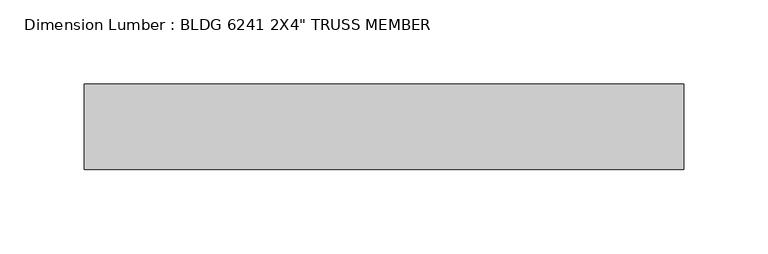
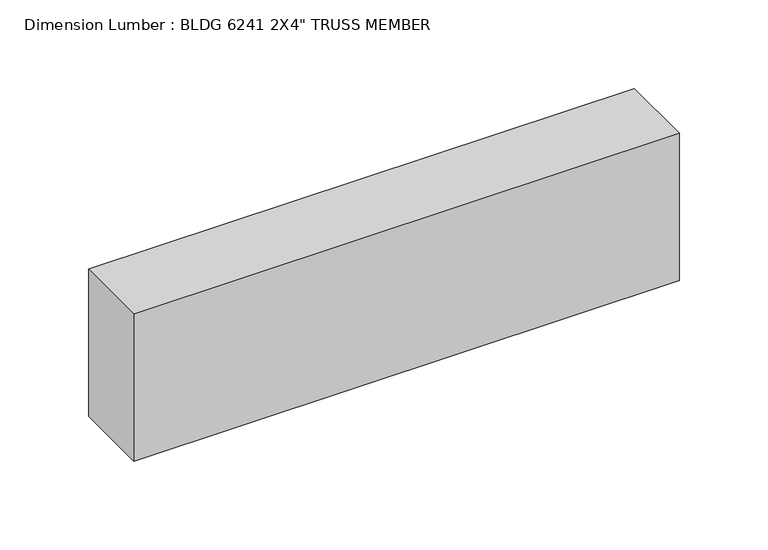
"""IFC4 building model written with IfcOpenShell, lengths in millimetres: beam geometry."""

from ifc_helpers import new_model, si_unit, frame, origin, place, context, project, spatial, polyline, outline, extrude, source, transform, mapped, element, save


def beam_7aad778a(model_context):
    return source(origin(), model_context, "Body", "SweptSolid", [
        extrude(outline(polyline([(307.975, -25.4), (-47.625, -25.4), (-47.625, 25.4), (307.975, 25.4), (307.975, -25.4)])), frame((0.0, 0.0, -50.8), z_axis=(0.0, 0.0, 1.0), x_axis=(1.0, 0.0, 0.0)), (0.0, 0.0, 1.0), 101.6),
    ])


if __name__ == "__main__":
    model = new_model("IFC4")
    model_context = context("Model", 3, world=origin())
    ifc_project = project(units=[si_unit("LENGTHUNIT", "METRE", prefix="MILLI")], contexts=[model_context])
    site = spatial("IfcSite", under=ifc_project)
    building = spatial("IfcBuilding", under=site)
    placement = place(None, origin())
    beam_shape = beam_7aad778a(model_context)
    element("IfcBeam", 1, ObjectType="Dimension Lumber : BLDG 6241 2X4\" TRUSS MEMBER", at=placement, inside=building, context=model_context, shape_type="MappedRepresentation", body=[
        mapped(beam_shape, transform((0.0, 0.0, 0.0), x_axis=(1.0, 0.0, 0.0), y_axis=(0.0, 1.0, 0.0), z_axis=(0.0, 0.0, 1.0))),
    ])
    save(model, "model.ifc")

# Revit data of these elements
# Type "Dimension Lumber : BLDG 6241 2X4\" TRUSS MEMBER"
#   Assembly Code = "B10"
#   A = 0.273472 SF
#   Length [instance default] = 5' - 0"
#   b = 0' - 2"
#   d = 0' - 4"
#   Structural Material [instance default] = Softwood, Lumber
# Element 1 (IfcBeam, "Dimension Lumber : BLDG 6241 2X4\" TRUSS MEMBER")
#   Materials on its faces: "Softwood, Lumber"
# Materials
#   "Softwood, Lumber": class "Wood", colour RGB 223 192 134, transparency 0, Description = "Pinus Echinata", Cost = 0
